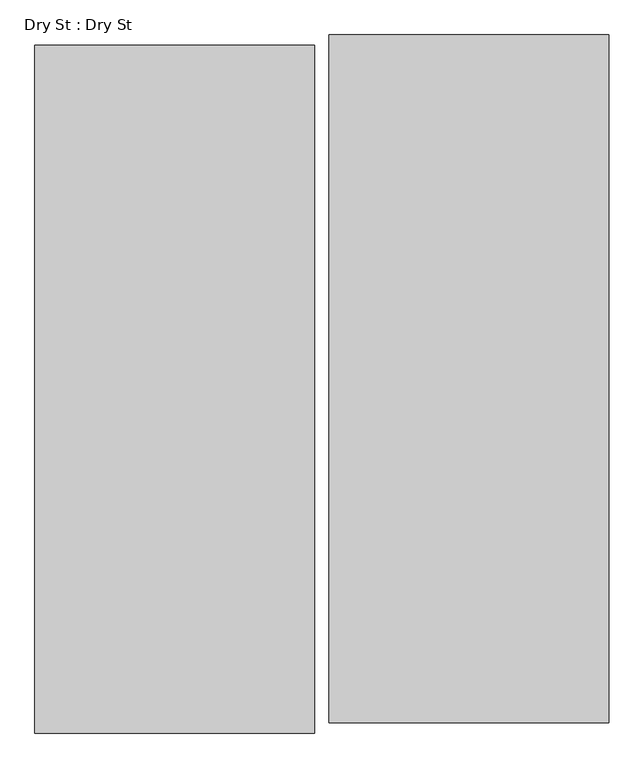
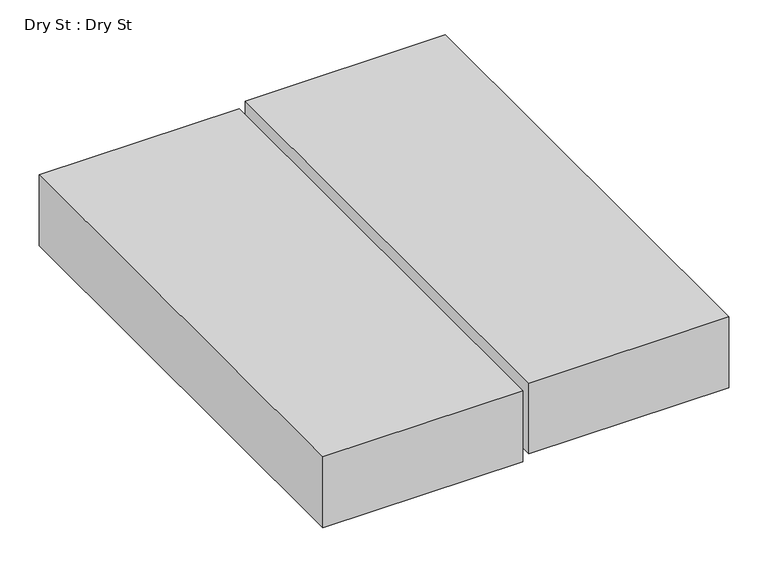
"""IFC4 building model written with IfcOpenShell, lengths in millimetres: geographic element geometry, Dry St : Dry St."""

from ifc_helpers import new_model, si_unit, origin, origin_with_axes, place, context, project, spatial, polyline, outline, extrude, source, transform, mapped, element, save


def dry_st_dry_st_2484704b(model_context):
    return source(origin(), model_context, "Body", "SweptSolid", [
        extrude(outline(polyline([(37769.9543265, 9894.5615366), (35331.5543265, 9894.5615366), (35331.5543265, 15888.9615366), (37769.9543265, 15888.9615366), (37769.9543265, 9894.5615366)])), origin_with_axes(), (0.0, 0.0, 1.0), 914.4),
        extrude(outline(polyline([(35205.1870052, 9805.6615366), (32766.7870052, 9805.6615366), (32766.7870052, 15800.0615366), (35205.1870052, 15800.0615366), (35205.1870052, 9805.6615366)])), origin_with_axes(), (0.0, 0.0, 1.0), 914.4),
    ])


if __name__ == "__main__":
    model = new_model("IFC4")
    model_context = context("Model", 3, world=origin())
    ifc_project = project(units=[si_unit("LENGTHUNIT", "METRE", prefix="MILLI")], contexts=[model_context])
    site = spatial("IfcSite", under=ifc_project)
    building = spatial("IfcBuilding", under=site)
    placement = place(None, origin())
    dry_st_dry_st_shape = dry_st_dry_st_2484704b(model_context)
    element("IfcGeographicElement", 1, ObjectType="Dry St : Dry St", at=placement, inside=building, context=model_context, shape_type="MappedRepresentation", body=[
        mapped(dry_st_dry_st_shape, transform((0.0, 0.0, 0.0), x_axis=(1.0, 0.0, 0.0), y_axis=(0.0, 1.0, 0.0), z_axis=(0.0, 0.0, 1.0))),
    ])
    save(model, "model.ifc")
